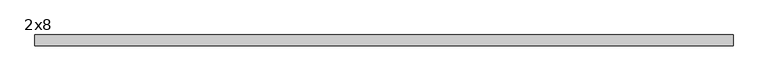
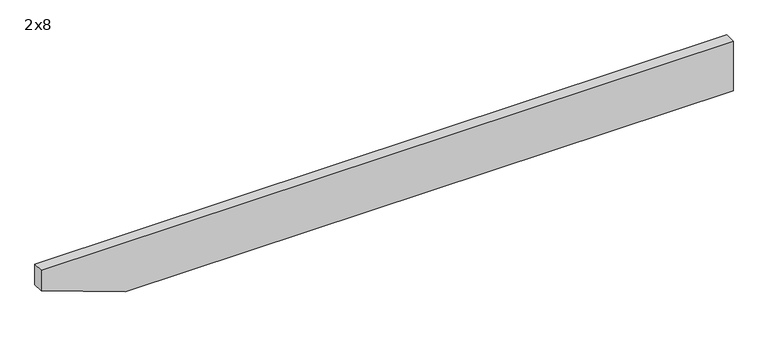
"""IFC4 building model written with IfcOpenShell, lengths in millimetres: beam geometry, Dimension Lumber - Truncated : 2x8."""

import ifcopenshell
import ifcopenshell.guid

model = None  # the IFC model being written
_history = None  # IfcOwnerHistory: only IFC2X3 demands one
_inside = {}  # id of a spatial element -> (the spatial element, [elements in it])
_under = {}  # id of a project, library or spatial element -> (it, [spatial elements below it])
_declared = {}  # id of a project -> (the project, [libraries it declares])
_typed = {}  # id of a type object -> (the type object, [elements of that type])
_made_of = {}  # id of a material, layer set ... -> (it, [elements and type objects made of it])


def new_model(schema):
    """Start an empty IFC model of exactly this schema.

    Asked for "IFC4X3", IfcOpenShell would pick the latest addendum, in which some entities
    have other attributes; the version numbers below select the first issue.
    IFC2X3 requires an IfcOwnerHistory on every rooted entity: one is made here for all.
    """
    global model, _history
    if schema == "IFC4X3":
        model = ifcopenshell.file(schema_version=(4, 3, 0, 0))
    else:
        model = ifcopenshell.file(schema=schema)
    _inside.clear()
    _under.clear()
    _declared.clear()
    _typed.clear()
    _made_of.clear()
    _history = None
    if model.schema == "IFC2X3":
        org = make("IfcOrganization", Name="unknown")
        user = make(
            "IfcPersonAndOrganization",
            ThePerson=make("IfcPerson", FamilyName="unknown"),
            TheOrganization=org,
        )
        app = make(
            "IfcApplication",
            ApplicationDeveloper=org,
            Version="unknown",
            ApplicationFullName="unknown",
            ApplicationIdentifier="unknown",
        )
        _history = make(
            "IfcOwnerHistory",
            OwningUser=user,
            OwningApplication=app,
            ChangeAction="ADDED",
            CreationDate=0,
        )
    return model


def make(cls, **values):
    """One entity of the class cls with the attributes given. An attribute that is None is left unset."""
    return model.create_entity(
        cls, **{name: value for name, value in values.items() if value is not None}
    )


def rooted(cls, **values):
    """An entity with a GlobalId (a new one), such as an element, a storey or a relation."""
    return make(cls, GlobalId=ifcopenshell.guid.new(), OwnerHistory=_history, **values)


def si_unit(unit_type, name, prefix=None):
    """IfcSIUnit, for example si_unit("LENGTHUNIT", "METRE", prefix="MILLI")."""
    return make("IfcSIUnit", UnitType=unit_type, Prefix=prefix, Name=name)


def assignment(units):
    """IfcUnitAssignment: the units of a project."""
    return None if units is None else make("IfcUnitAssignment", Units=units)


def point(xyz):
    """IfcCartesianPoint."""
    return None if xyz is None else make("IfcCartesianPoint", Coordinates=xyz)


def direction(xyz):
    """IfcDirection."""
    return None if xyz is None else make("IfcDirection", DirectionRatios=xyz)


def frame(location, z_axis=None, x_axis=None):
    """IfcAxis2Placement3D, a coordinate frame: its origin and axes. An axis left out is left unset."""
    return make(
        "IfcAxis2Placement3D",
        Location=point(location),
        Axis=direction(z_axis),
        RefDirection=direction(x_axis),
    )


def origin():
    """The frame at (0, 0, 0) with its axes left unset."""
    return frame((0.0, 0.0, 0.0))


def place(relative_to, where):
    """IfcLocalPlacement: puts the frame where relative to a parent placement (None: the world)."""
    return make(
        "IfcLocalPlacement", PlacementRelTo=relative_to, RelativePlacement=where
    )


def context(
    kind, dimensions, precision=None, world=None, true_north=None, identifier=None
):
    """IfcGeometricRepresentationContext, for example the 3D "Model" context."""
    return make(
        "IfcGeometricRepresentationContext",
        ContextIdentifier=identifier,
        ContextType=kind,
        CoordinateSpaceDimension=dimensions,
        Precision=precision,
        WorldCoordinateSystem=world,
        TrueNorth=true_north,
    )


def project(units=None, contexts=None):
    """IfcProject with its units and contexts."""
    return rooted(
        "IfcProject",
        Name="project",
        RepresentationContexts=contexts,
        UnitsInContext=assignment(units),
    )


def spatial(cls, under=None, at=None, **own):
    """A site, building, storey or space (cls), placed at a placement, below another one or the project."""
    s = rooted(cls, ObjectPlacement=at, **own)
    if under is not None:
        _under.setdefault(under.id(), (under, []))[1].append(s)
    return s


def polyline(points):
    """IfcPolyline through the points."""
    return make("IfcPolyline", Points=[point(p) for p in points])


def outline(outer, holes=None, kind="AREA"):
    """IfcArbitraryClosedProfileDef: a profile drawn as a closed curve; with holes, ...WithVoids."""
    if holes is None:
        return make("IfcArbitraryClosedProfileDef", ProfileType=kind, OuterCurve=outer)
    return make(
        "IfcArbitraryProfileDefWithVoids",
        ProfileType=kind,
        OuterCurve=outer,
        InnerCurves=holes,
    )


def extrude(swept, where, along, depth):
    """IfcExtrudedAreaSolid: the profile swept, set in the frame where, extruded along a direction by depth."""
    return make(
        "IfcExtrudedAreaSolid",
        SweptArea=swept,
        Position=where,
        ExtrudedDirection=direction(along),
        Depth=depth,
    )


def shape(context_of_items, identifier, shape_type, items):
    """IfcShapeRepresentation: the items that make up one representation, for example the "Body"."""
    return make(
        "IfcShapeRepresentation",
        ContextOfItems=context_of_items,
        RepresentationIdentifier=identifier,
        RepresentationType=shape_type,
        Items=items,
    )


def source(mapping_origin, context_of_items, identifier, shape_type, items):
    """IfcRepresentationMap: a shape defined once, which mapped items show again and again."""
    return make(
        "IfcRepresentationMap",
        MappingOrigin=mapping_origin,
        MappedRepresentation=shape(context_of_items, identifier, shape_type, items),
    )


def transform(
    local_origin,
    x_axis=None,
    y_axis=None,
    z_axis=None,
    scale=None,
    scale2=None,
    scale3=None,
    uniform=True,
):
    """IfcCartesianTransformationOperator3D, or its non-uniform kind. x_axis, y_axis, z_axis: its Axis1, 2, 3."""
    if uniform:
        return make(
            "IfcCartesianTransformationOperator3D",
            Axis1=direction(x_axis),
            Axis2=direction(y_axis),
            LocalOrigin=point(local_origin),
            Scale=scale,
            Axis3=direction(z_axis),
        )
    return make(
        "IfcCartesianTransformationOperator3DnonUniform",
        Axis1=direction(x_axis),
        Axis2=direction(y_axis),
        LocalOrigin=point(local_origin),
        Scale=scale,
        Axis3=direction(z_axis),
        Scale2=scale2,
        Scale3=scale3,
    )


def mapped(mapping_source, mapping_target):
    """IfcMappedItem: shows the shape of a source again, moved by a transform."""
    return make(
        "IfcMappedItem", MappingSource=mapping_source, MappingTarget=mapping_target
    )


def made_of(thing, what):
    """Note that an element or type object is made of a material, layer set ...; save() writes the relation."""
    if what is not None:
        _made_of.setdefault(what.id(), (what, []))[1].append(thing)
    return thing


def element(
    cls,
    number,
    at=None,
    inside=None,
    cuts=None,
    type_object=None,
    material=None,
    context=None,
    identifier="Body",
    shape_type=None,
    held_by="IfcProductDefinitionShape",
    body=None,
    shapes=None,
    **own,
):
    """One element of the class cls, such as IfcWall. Its Tag is "e" and its number.

    at: its placement. inside: the storey or other place that contains it. cuts: it is an
    opening in that element (IfcRelVoidsElement). A single representation is given by context,
    identifier, shape_type and body (its items); several are given by shapes. held_by: the class
    of the entity that holds the representations. save() writes the other relations.
    """
    e = rooted(cls, Tag="e%d" % number, ObjectPlacement=at, **own)
    if body is not None:
        shapes = [shape(context, identifier, shape_type, body)]
    if shapes is not None:
        e.Representation = make(held_by, Representations=shapes)
    if inside is not None:
        _inside.setdefault(inside.id(), (inside, []))[1].append(e)
    if cuts is not None:
        rooted(
            "IfcRelVoidsElement", RelatingBuildingElement=cuts, RelatedOpeningElement=e
        )
    if type_object is not None:
        _typed.setdefault(type_object.id(), (type_object, []))[1].append(e)
    return made_of(e, material)


def aggregate(whole, parts):
    """IfcRelAggregates: a whole, such as a stair, and the parts it consists of."""
    return rooted("IfcRelAggregates", RelatingObject=whole, RelatedObjects=parts)


def save(model, path):
    """Write the relations noted so far, then the file.

    IfcRelAggregates (storeys below a building ...), IfcRelContainedInSpatialStructure (elements
    in a storey), IfcRelDefinesByType, IfcRelAssociatesMaterial and IfcRelDeclares: one each for
    every whole, place, type object, material and project.
    """
    for whole, parts in _under.values():
        aggregate(whole, parts)
    for where, things in _inside.values():
        rooted(
            "IfcRelContainedInSpatialStructure",
            RelatedElements=things,
            RelatingStructure=where,
        )
    for kind, things in _typed.values():
        rooted("IfcRelDefinesByType", RelatedObjects=things, RelatingType=kind)
    for what, things in _made_of.values():
        rooted("IfcRelAssociatesMaterial", RelatedObjects=things, RelatingMaterial=what)
    for by, libraries in _declared.values():
        rooted("IfcRelDeclares", RelatingContext=by, RelatedDefinitions=libraries)
    model.write(path)


def beam_2x8_64904455(model_context):
    return source(origin(), model_context, "Body", "SweptSolid", [
        extrude(outline(polyline([(-92.075, 1219.2), (92.075, 1219.2), (92.075, -1219.2), (15.875, -1219.2), (-92.075, -922.6098126), (-92.075, 1219.2)])), frame((0.0, -19.05, 0.0), z_axis=(0.0, 1.0, 0.0), x_axis=(0.0, 0.0, 1.0)), (0.0, 0.0, 1.0), 38.1),
    ])


if __name__ == "__main__":
    model = new_model("IFC4")
    model_context = context("Model", 3, world=origin())
    ifc_project = project(units=[si_unit("LENGTHUNIT", "METRE", prefix="MILLI")], contexts=[model_context])
    site = spatial("IfcSite", under=ifc_project)
    building = spatial("IfcBuilding", under=site)
    placement = place(None, origin())
    beam_2x8_shape = beam_2x8_64904455(model_context)
    element("IfcBeam", 1, ObjectType="Dimension Lumber - Truncated : 2x8", at=placement, inside=building, context=model_context, shape_type="MappedRepresentation", body=[
        mapped(beam_2x8_shape, transform((0.0, 0.0, 0.0), x_axis=(1.0, 0.0, 0.0), y_axis=(0.0, 1.0, 0.0), z_axis=(0.0, 0.0, 1.0))),
    ])
    save(model, "model.ifc")

# Revit data of these elements
# Type "Dimension Lumber - Truncated : 2x8"
#   Assembly Code = "B10"
#   Leading Edge Dimension = 0' - 3"
#   Start Angle = 70.00°
#   End Angle = 0.00°
#   A = 0.0755556 SF
#   Length [instance default] = 5' - 0"
#   b = 0' - 1 1/2"
#   d = 0' - 7 1/4"
#   Structural Material = Softwood, Lumber - hortz
# Element 1 (IfcBeam, "Dimension Lumber - Truncated : 2x8")
#   Materials on its faces: "Softwood, Lumber - hortz"
# Materials
#   "Softwood, Lumber - hortz": class "Wood", colour RGB 131 91 56, transparency 0, Description = "Pinus Echinata", Cost = 0
